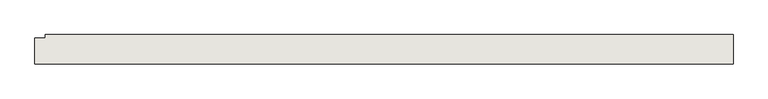
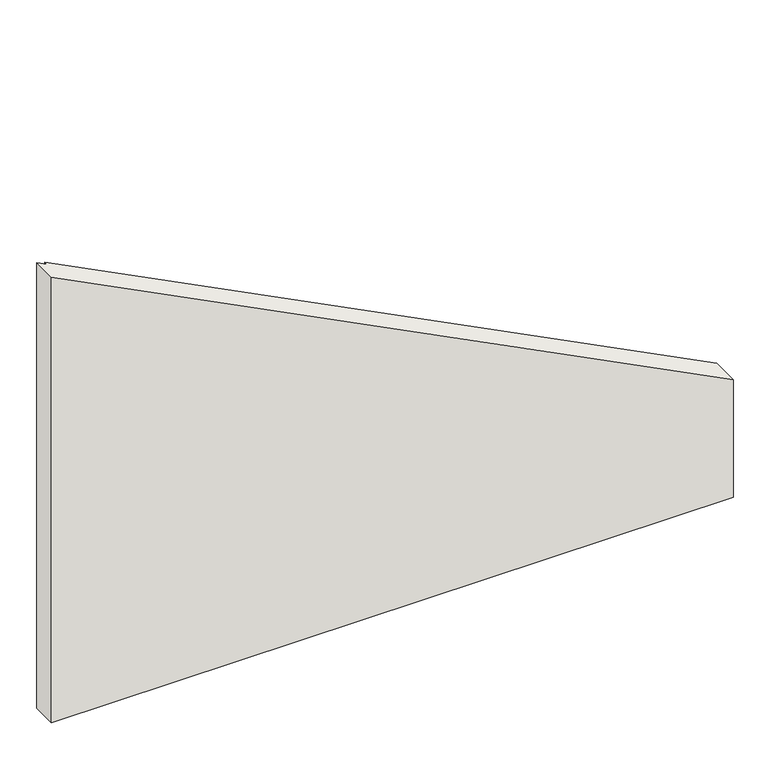
"""IFC4 building model written with IfcOpenShell, lengths in millimetres: wall geometry, Holzwand."""

from ifc_helpers import new_model, si_unit, origin, place, context, project, spatial, faceted_brep, source, transform, mapped, element, save


def wall_e5cfdf7a(model_context):
    return source(origin(), model_context, "Body", "Brep", [
        faceted_brep([(0.0, 176.0, 3283.5797924), (0.0, 0.0, 3283.5797924), (4750.0, 0.0, 863.3339073), (4750.0, 200.0, 863.3339073), (70.0, 200.0, 3247.913011), (70.0, 176.0, 3247.913011), (4750.0, 200.0, 0.0), (70.0, 200.0, 0.0), (4750.0, 0.0, 0.0), (0.0, 0.0, 0.0), (0.0, 176.0, 0.0), (70.0, 176.0, 0.0)], [[[0, 1, 2, 3, 4, 5]], [[4, 3, 6, 7]], [[3, 2, 8, 6]], [[2, 1, 9, 8]], [[10, 9, 1, 0]], [[0, 5, 11, 10]], [[5, 4, 7, 11]], [[8, 9, 10, 11, 7, 6]]]),
    ])


if __name__ == "__main__":
    model = new_model("IFC4")
    model_context = context("Model", 3, world=origin())
    ifc_project = project(units=[si_unit("LENGTHUNIT", "METRE", prefix="MILLI")], contexts=[model_context])
    site = spatial("IfcSite", under=ifc_project)
    building = spatial("IfcBuilding", under=site)
    placement = place(None, origin())
    wall_shape = wall_e5cfdf7a(model_context)
    element("IfcWall", 1, ObjectType="Holzwand", at=placement, inside=building, context=model_context, shape_type="MappedRepresentation", body=[
        mapped(wall_shape, transform((0.0, 0.0, 0.0), x_axis=(1.0, 0.0, 0.0), y_axis=(0.0, 1.0, 0.0), z_axis=(0.0, 0.0, 1.0))),
    ])
    save(model, "model.ifc")

# Revit data of these elements
# Element 1 (IfcWall, "Holzwand")
#   Materials on its faces: "holzschalung"
# Materials
#   "holzschalung": class "Unassigned", colour RGB 128 128 128, transparency 0
